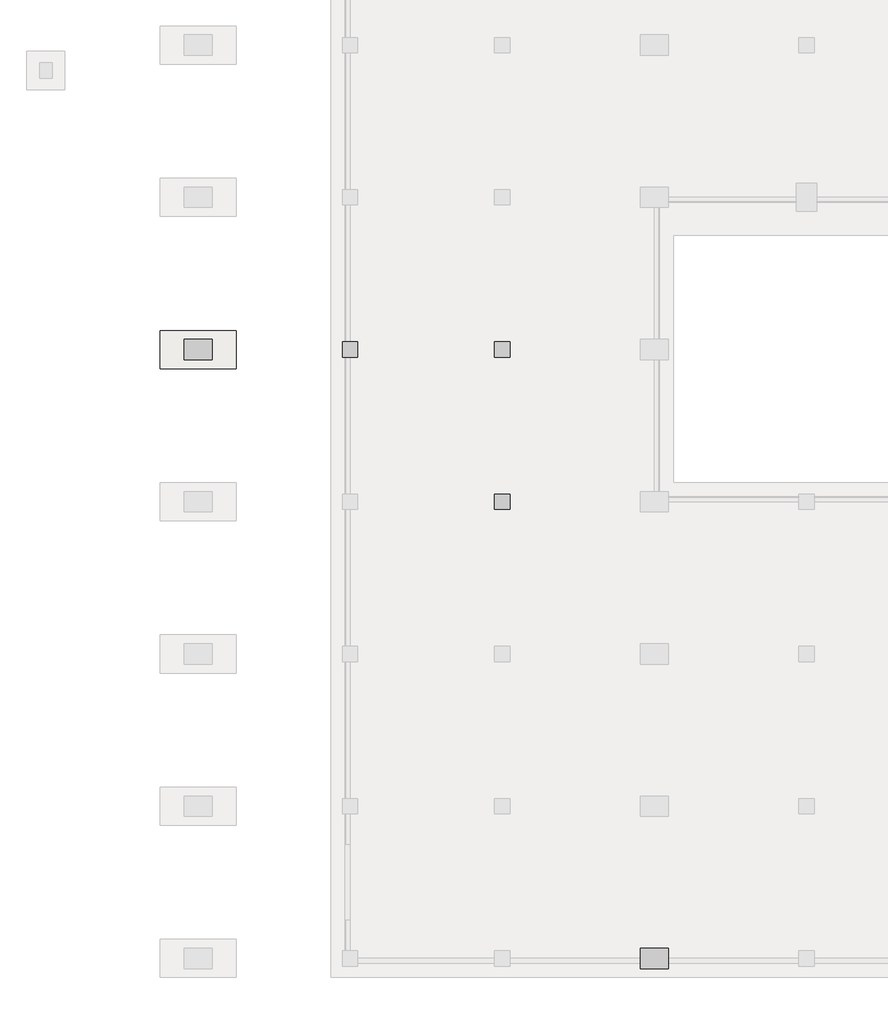
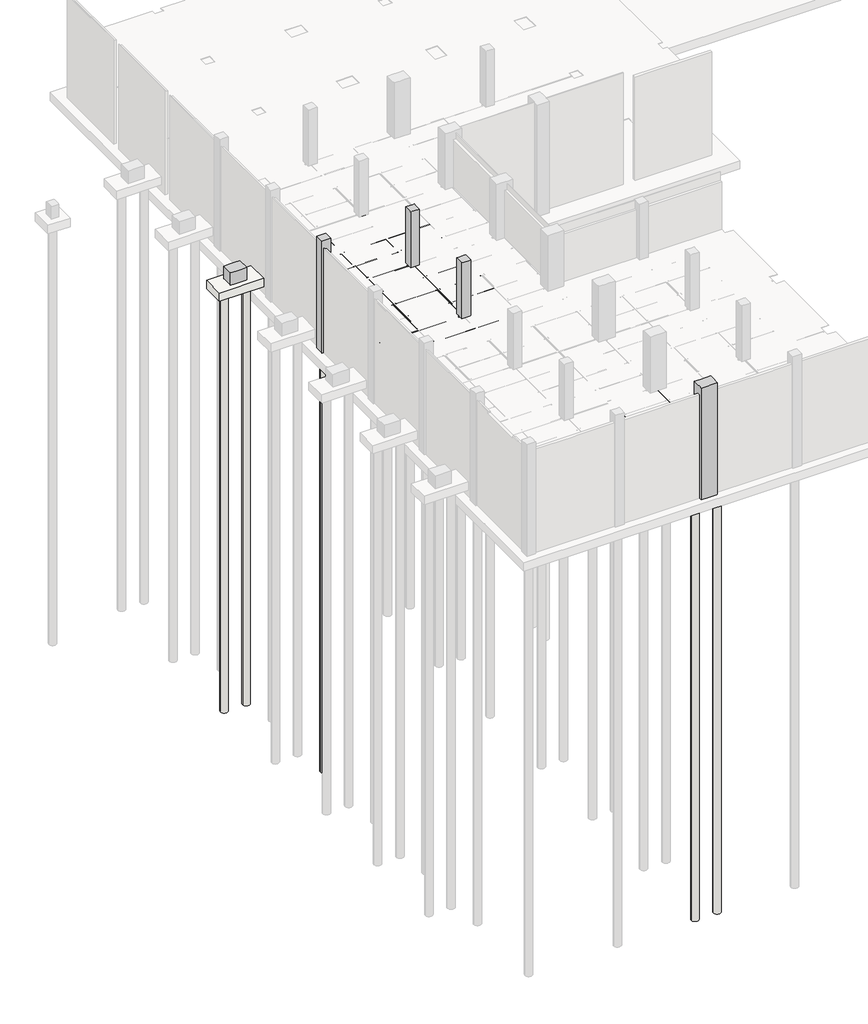
# Not in any storey, part 3 of 16: 28 beams, 6 slabs, 5 columns.
# Revit data of these elements (continued)
# Element 34 (IfcSlab, "Foundation Rectangular (Non-Pile) : H_SF_AR_S18_Shallow Fdn_Bitumen_1500x3000xT600_F1")
#   Comments = ""
#   Structural Material = 00_Concrete_Reinf. Conc.
#   Phase Created = New Construction
#   Materials on its faces: "00_Concrete_Reinf. Conc."
# Elements 35, 36 (IfcSlab, "PILE : H_SF_AR_S19_PHC Pile_Pre-boring_D500_L30")
#   Structural Material = Concrete, Precast
#   Phase Created = New Construction
#   Materials on its faces: "Concrete, Precast"
# Elements 37, 38, 39 (IfcSlab, "PILE : H_SF_AR_S19_PHC Pile_Pre-boring_D500_L30")
#   Structural Material = none
#   Phase Created = New Construction
# Materials
#   "Steel, 45-345": class "Metal", colour RGB 189 187 185, transparency 0, Description = "Steel 345 MPa", Cost = 0
#   "00_Concrete_Reinf. Conc.": class "Concrete", colour RGB 176 176 176, transparency 0, Description = "Reinf. Conc.", Cost = 0, Image = Concrete.Cast-In-Place.Flat.Polished.Grey.jpg
#   "Concrete, Precast": class "Concrete", colour RGB 115 116 108, transparency 0, Description = "Precast concrete", Cost = 0
